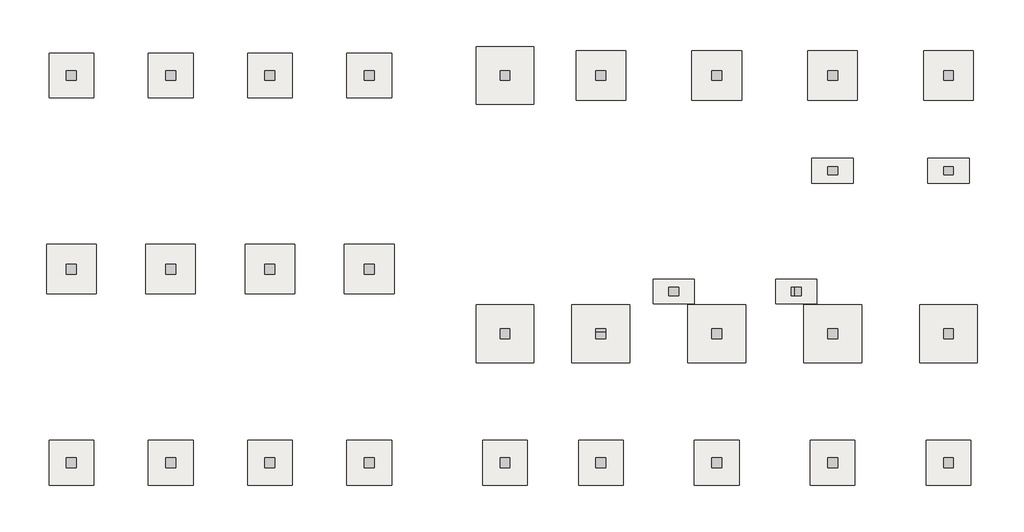
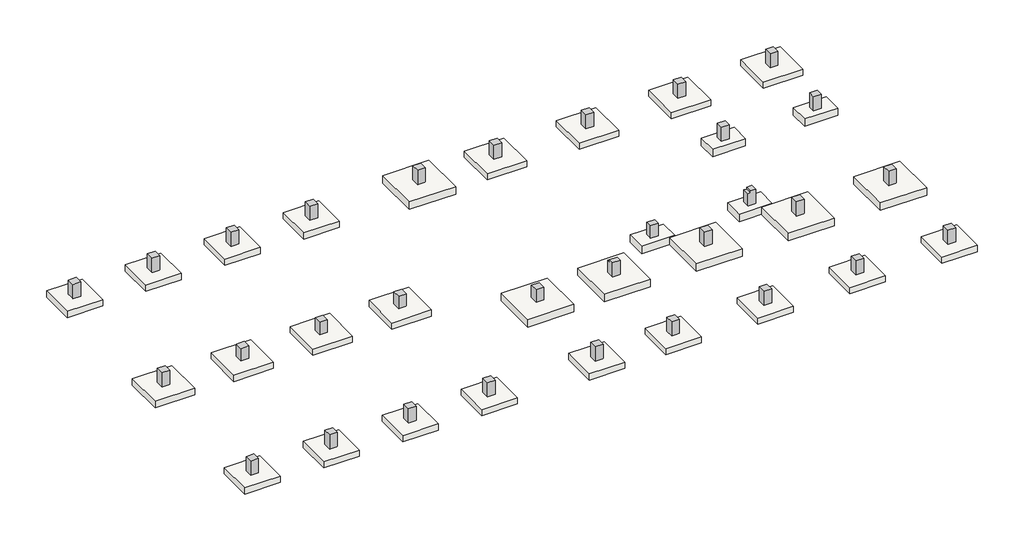
# Not in any storey: 31 columns, 31 slabs.
"""IFC4 building model written with IfcOpenShell, lengths in millimetres."""

import ifcopenshell
import ifcopenshell.guid

model = None  # the IFC model being written
_history = None  # IfcOwnerHistory: only IFC2X3 demands one
_inside = {}  # id of a spatial element -> (the spatial element, [elements in it])
_under = {}  # id of a project, library or spatial element -> (it, [spatial elements below it])
_declared = {}  # id of a project -> (the project, [libraries it declares])
_typed = {}  # id of a type object -> (the type object, [elements of that type])
_made_of = {}  # id of a material, layer set ... -> (it, [elements and type objects made of it])


def new_model(schema):
    """Start an empty IFC model of exactly this schema.

    Asked for "IFC4X3", IfcOpenShell would pick the latest addendum, in which some entities
    have other attributes; the version numbers below select the first issue.
    IFC2X3 requires an IfcOwnerHistory on every rooted entity: one is made here for all.
    """
    global model, _history
    if schema == "IFC4X3":
        model = ifcopenshell.file(schema_version=(4, 3, 0, 0))
    else:
        model = ifcopenshell.file(schema=schema)
    _inside.clear()
    _under.clear()
    _declared.clear()
    _typed.clear()
    _made_of.clear()
    _history = None
    if model.schema == "IFC2X3":
        org = make("IfcOrganization", Name="unknown")
        user = make(
            "IfcPersonAndOrganization",
            ThePerson=make("IfcPerson", FamilyName="unknown"),
            TheOrganization=org,
        )
        app = make(
            "IfcApplication",
            ApplicationDeveloper=org,
            Version="unknown",
            ApplicationFullName="unknown",
            ApplicationIdentifier="unknown",
        )
        _history = make(
            "IfcOwnerHistory",
            OwningUser=user,
            OwningApplication=app,
            ChangeAction="ADDED",
            CreationDate=0,
        )
    return model


def make(cls, **values):
    """One entity of the class cls with the attributes given. An attribute that is None is left unset."""
    return model.create_entity(
        cls, **{name: value for name, value in values.items() if value is not None}
    )


def rooted(cls, **values):
    """An entity with a GlobalId (a new one), such as an element, a storey or a relation."""
    return make(cls, GlobalId=ifcopenshell.guid.new(), OwnerHistory=_history, **values)


def si_unit(unit_type, name, prefix=None):
    """IfcSIUnit, for example si_unit("LENGTHUNIT", "METRE", prefix="MILLI")."""
    return make("IfcSIUnit", UnitType=unit_type, Prefix=prefix, Name=name)


def assignment(units):
    """IfcUnitAssignment: the units of a project."""
    return None if units is None else make("IfcUnitAssignment", Units=units)


def point(xyz):
    """IfcCartesianPoint."""
    return None if xyz is None else make("IfcCartesianPoint", Coordinates=xyz)


def direction(xyz):
    """IfcDirection."""
    return None if xyz is None else make("IfcDirection", DirectionRatios=xyz)


def frame(location, z_axis=None, x_axis=None):
    """IfcAxis2Placement3D, a coordinate frame: its origin and axes. An axis left out is left unset."""
    return make(
        "IfcAxis2Placement3D",
        Location=point(location),
        Axis=direction(z_axis),
        RefDirection=direction(x_axis),
    )


def origin():
    """The frame at (0, 0, 0) with its axes left unset."""
    return frame((0.0, 0.0, 0.0))


def place(relative_to, where):
    """IfcLocalPlacement: puts the frame where relative to a parent placement (None: the world)."""
    return make(
        "IfcLocalPlacement", PlacementRelTo=relative_to, RelativePlacement=where
    )


def context(
    kind, dimensions, precision=None, world=None, true_north=None, identifier=None
):
    """IfcGeometricRepresentationContext, for example the 3D "Model" context."""
    return make(
        "IfcGeometricRepresentationContext",
        ContextIdentifier=identifier,
        ContextType=kind,
        CoordinateSpaceDimension=dimensions,
        Precision=precision,
        WorldCoordinateSystem=world,
        TrueNorth=true_north,
    )


def project(units=None, contexts=None):
    """IfcProject with its units and contexts."""
    return rooted(
        "IfcProject",
        Name="project",
        RepresentationContexts=contexts,
        UnitsInContext=assignment(units),
    )


def spatial(cls, under=None, at=None, **own):
    """A site, building, storey or space (cls), placed at a placement, below another one or the project."""
    s = rooted(cls, ObjectPlacement=at, **own)
    if under is not None:
        _under.setdefault(under.id(), (under, []))[1].append(s)
    return s


def polyline(points):
    """IfcPolyline through the points."""
    return make("IfcPolyline", Points=[point(p) for p in points])


def outline(outer, holes=None, kind="AREA"):
    """IfcArbitraryClosedProfileDef: a profile drawn as a closed curve; with holes, ...WithVoids."""
    if holes is None:
        return make("IfcArbitraryClosedProfileDef", ProfileType=kind, OuterCurve=outer)
    return make(
        "IfcArbitraryProfileDefWithVoids",
        ProfileType=kind,
        OuterCurve=outer,
        InnerCurves=holes,
    )


def extrude(swept, where, along, depth):
    """IfcExtrudedAreaSolid: the profile swept, set in the frame where, extruded along a direction by depth."""
    return make(
        "IfcExtrudedAreaSolid",
        SweptArea=swept,
        Position=where,
        ExtrudedDirection=direction(along),
        Depth=depth,
    )


def faces_of(points, faces, orient=None, outer=None):
    """IfcFace entities. A face is a list of loops; a loop is a list of indices into points, from 0.

    orient and outer hold one flag for each loop. By default every Orientation is true, the
    first loop of a face is its IfcFaceOuterBound and the others are IfcFaceBound.
    """
    made = []
    for i, loops in enumerate(faces):
        bounds = []
        for j, loop in enumerate(loops):
            is_outer = j == 0 if outer is None else outer[i][j]
            bounds.append(
                make(
                    "IfcFaceOuterBound" if is_outer else "IfcFaceBound",
                    Bound=make("IfcPolyLoop", Polygon=[points[k] for k in loop]),
                    Orientation=True if orient is None else orient[i][j],
                )
            )
        made.append(make("IfcFace", Bounds=bounds))
    return made


def faceted_brep(points, faces, orient=None, outer=None, voids=None):
    """IfcFacetedBrep: a solid bounded by flat faces; with voids (closed shells), ...WithVoids."""
    shared = [point(p) for p in points]
    hull = make("IfcClosedShell", CfsFaces=faces_of(shared, faces, orient, outer))
    if voids is None:
        return make("IfcFacetedBrep", Outer=hull)
    return make(
        "IfcFacetedBrepWithVoids",
        Outer=hull,
        Voids=[
            make(cls, CfsFaces=faces_of(shared, fs, o, b)) for cls, fs, o, b in voids
        ],
    )


def shape(context_of_items, identifier, shape_type, items):
    """IfcShapeRepresentation: the items that make up one representation, for example the "Body"."""
    return make(
        "IfcShapeRepresentation",
        ContextOfItems=context_of_items,
        RepresentationIdentifier=identifier,
        RepresentationType=shape_type,
        Items=items,
    )


def made_of(thing, what):
    """Note that an element or type object is made of a material, layer set ...; save() writes the relation."""
    if what is not None:
        _made_of.setdefault(what.id(), (what, []))[1].append(thing)
    return thing


def element(
    cls,
    number,
    at=None,
    inside=None,
    cuts=None,
    type_object=None,
    material=None,
    context=None,
    identifier="Body",
    shape_type=None,
    held_by="IfcProductDefinitionShape",
    body=None,
    shapes=None,
    **own,
):
    """One element of the class cls, such as IfcWall. Its Tag is "e" and its number.

    at: its placement. inside: the storey or other place that contains it. cuts: it is an
    opening in that element (IfcRelVoidsElement). A single representation is given by context,
    identifier, shape_type and body (its items); several are given by shapes. held_by: the class
    of the entity that holds the representations. save() writes the other relations.
    """
    e = rooted(cls, Tag="e%d" % number, ObjectPlacement=at, **own)
    if body is not None:
        shapes = [shape(context, identifier, shape_type, body)]
    if shapes is not None:
        e.Representation = make(held_by, Representations=shapes)
    if inside is not None:
        _inside.setdefault(inside.id(), (inside, []))[1].append(e)
    if cuts is not None:
        rooted(
            "IfcRelVoidsElement", RelatingBuildingElement=cuts, RelatedOpeningElement=e
        )
    if type_object is not None:
        _typed.setdefault(type_object.id(), (type_object, []))[1].append(e)
    return made_of(e, material)


def aggregate(whole, parts):
    """IfcRelAggregates: a whole, such as a stair, and the parts it consists of."""
    return rooted("IfcRelAggregates", RelatingObject=whole, RelatedObjects=parts)


def save(model, path):
    """Write the relations noted so far, then the file.

    IfcRelAggregates (storeys below a building ...), IfcRelContainedInSpatialStructure (elements
    in a storey), IfcRelDefinesByType, IfcRelAssociatesMaterial and IfcRelDeclares: one each for
    every whole, place, type object, material and project.
    """
    for whole, parts in _under.values():
        aggregate(whole, parts)
    for where, things in _inside.values():
        rooted(
            "IfcRelContainedInSpatialStructure",
            RelatedElements=things,
            RelatingStructure=where,
        )
    for kind, things in _typed.values():
        rooted("IfcRelDefinesByType", RelatedObjects=things, RelatingType=kind)
    for what, things in _made_of.values():
        rooted("IfcRelAssociatesMaterial", RelatedObjects=things, RelatingMaterial=what)
    for by, libraries in _declared.values():
        rooted("IfcRelDeclares", RelatingContext=by, RelatedDefinitions=libraries)
    model.write(path)


model = new_model("IFC4")

# Units and contexts
model_context = context("Model", 3, world=origin())
ifc_project = project(units=[si_unit("LENGTHUNIT", "METRE", prefix="MILLI")], contexts=[model_context])

# Site, building
site = spatial("IfcSite", under=ifc_project)
building = spatial("IfcBuilding", under=site)

# Columns
placement = place(None, origin())
element("IfcColumn", 1, ObjectType="RC_Column_Rectangular : H_SC_AR_S15_UG PED_W600xL600_Bit", at=placement, inside=building, context=model_context, shape_type="Brep", body=[
    faceted_brep([(300.0, 12499.5208589, -1000.0381366), (300.0, 11899.5208589, -1000.0381366), (-300.0, 11899.5208589, -1000.0381366), (-300.0, 12499.5208589, -1000.0381366), (300.0, 12499.5208589, 149.9618634), (300.0, 11899.5208589, 149.9618634), (300.0, 11899.5208589, -0.0381366), (300.0, 11899.5208589, -500.0381366), (300.0, 12499.5208589, -500.0381366), (300.0, 12499.5208589, -0.0381366), (-300.0, 11899.5208589, 149.9618634), (-300.0, 11899.5208589, -0.0381366), (-300.0, 11899.5208589, -500.0381366), (-300.0, 12499.5208589, 149.9618634), (-300.0, 12499.5208589, -0.0381366), (-300.0, 12499.5208589, -500.0381366)], [[[0, 1, 2, 3]], [[4, 5, 6, 7, 1, 0, 8, 9]], [[5, 10, 11, 12, 2, 1, 7, 6]], [[10, 13, 14, 15, 3, 2, 12, 11]], [[13, 4, 9, 8, 0, 3, 15, 14]], [[4, 13, 10, 5]]]),
])
element("IfcColumn", 2, ObjectType="RC_Column_Rectangular : H_SC_AR_S15_UG PED_W600xL600_Bit", at=placement, inside=building, context=model_context, shape_type="SweptSolid", body=[
    extrude(outline(polyline([(6300.0, 12499.5208589), (6300.0, 11899.5208589), (5700.0, 11899.5208589), (5700.0, 12499.5208589), (6300.0, 12499.5208589)])), frame((0.0, 0.0, -1000.0381366), z_axis=(0.0, 0.0, 1.0), x_axis=(1.0, 0.0, 0.0)), (0.0, 0.0, 1.0), 1000.0),
])
element("IfcColumn", 3, ObjectType="RC_Column_Rectangular : H_SC_AR_S15_UG PED_W600xL600_Bit", at=placement, inside=building, context=model_context, shape_type="SweptSolid", body=[
    extrude(outline(polyline([(12300.0, 12499.5208589), (12300.0, 11899.5208589), (11700.0, 11899.5208589), (11700.0, 12499.5208589), (12300.0, 12499.5208589)])), frame((0.0, 0.0, -1000.0381366), z_axis=(0.0, 0.0, 1.0), x_axis=(1.0, 0.0, 0.0)), (0.0, 0.0, 1.0), 1000.0),
])
element("IfcColumn", 4, ObjectType="RC_Column_Rectangular : H_SC_AR_S15_UG PED_W600xL600_Bit", at=placement, inside=building, context=model_context, shape_type="Brep", body=[
    faceted_brep([(18300.0, 12499.5208589, -1000.0381366), (18300.0, 11899.5208589, -1000.0381366), (17700.0, 11899.5208589, -1000.0381366), (17700.0, 12499.5208589, -1000.0381366), (18300.0, 12499.5208589, -0.0381366), (18300.0, 11899.5208589, -0.0381366), (18200.0, 11899.5208589, -0.0381366), (17700.0, 11899.5208589, -0.0381366), (17700.0, 12499.5208589, -0.0381366)], [[[0, 1, 2, 3]], [[1, 0, 4, 5]], [[2, 1, 5, 6, 7]], [[3, 2, 7, 8]], [[0, 3, 8, 4]], [[5, 4, 8, 7, 6]]]),
])
element("IfcColumn", 5, ObjectType="RC_Column_Rectangular : H_SC_AR_S15_UG PED_W600xL600_Bit", at=placement, inside=building, context=model_context, shape_type="Brep", body=[
    faceted_brep([(300.0, 24199.5208589, -1000.0381366), (300.0, 23599.5208589, -1000.0381366), (-300.0, 23599.5208589, -1000.0381366), (-300.0, 24199.5208589, -1000.0381366), (300.0, 24199.5208589, 149.9618634), (300.0, 23599.5208589, 149.9618634), (300.0, 23599.5208589, -0.0381366), (300.0, 23599.5208589, -500.0381366), (300.0, 24199.5208589, -500.0381366), (300.0, 24199.5208589, -0.0381366), (-300.0, 23599.5208589, 149.9618634), (-300.0, 23599.5208589, -0.0381366), (-300.0, 23599.5208589, -500.0381366), (-300.0, 24199.5208589, 149.9618634)], [[[0, 1, 2, 3]], [[4, 5, 6, 7, 1, 0, 8, 9]], [[5, 10, 11, 12, 2, 1, 7, 6]], [[10, 13, 3, 2, 12, 11]], [[13, 4, 9, 8, 0, 3]], [[4, 13, 10, 5]]]),
])
element("IfcColumn", 6, ObjectType="RC_Column_Rectangular : H_SC_AR_S15_UG PED_W600xL600_Bit", at=placement, inside=building, context=model_context, shape_type="Brep", body=[
    faceted_brep([(6300.0, 24199.5208589, -1000.0381366), (6300.0, 23599.5208589, -1000.0381366), (5700.0, 23599.5208589, -1000.0381366), (5700.0, 24199.5208589, -1000.0381366), (6300.0, 24199.5208589, 149.9618634), (6300.0, 23599.5208589, 149.9618634), (6300.0, 23599.5208589, -0.0381366), (6300.0, 23599.5208589, -500.0381366), (6300.0, 24199.5208589, -500.0381366), (6300.0, 24199.5208589, -0.0381366), (5700.0, 23599.5208589, 149.9618634), (5700.0, 23599.5208589, -0.0381366), (5700.0, 23599.5208589, -500.0381366), (5700.0, 24199.5208589, 149.9618634), (5700.0, 24199.5208589, -0.0381366), (5700.0, 24199.5208589, -500.0381366)], [[[0, 1, 2, 3]], [[4, 5, 6, 7, 1, 0, 8, 9]], [[5, 10, 11, 12, 2, 1, 7, 6]], [[10, 13, 14, 15, 3, 2, 12, 11]], [[13, 4, 9, 8, 0, 3, 15, 14]], [[4, 13, 10, 5]]]),
])
element("IfcColumn", 7, ObjectType="RC_Column_Rectangular : H_SC_AR_S15_UG PED_W600xL600_Bit", at=placement, inside=building, context=model_context, shape_type="Brep", body=[
    faceted_brep([(12300.0, 24199.5208589, -1000.0381366), (12300.0, 23599.5208589, -1000.0381366), (11700.0, 23599.5208589, -1000.0381366), (11700.0, 24199.5208589, -1000.0381366), (12300.0, 24199.5208589, 149.9618634), (12300.0, 23599.5208589, 149.9618634), (12300.0, 23599.5208589, -0.0381366), (12300.0, 23599.5208589, -500.0381366), (12300.0, 24199.5208589, -500.0381366), (12300.0, 24199.5208589, -0.0381366), (11700.0, 23599.5208589, 149.9618634), (11700.0, 23599.5208589, -0.0381366), (11700.0, 23599.5208589, -500.0381366), (11700.0, 24199.5208589, 149.9618634), (11700.0, 24199.5208589, -0.0381366), (11700.0, 24199.5208589, -500.0381366)], [[[0, 1, 2, 3]], [[4, 5, 6, 7, 1, 0, 8, 9]], [[5, 10, 11, 12, 2, 1, 7, 6]], [[10, 13, 14, 15, 3, 2, 12, 11]], [[13, 4, 9, 8, 0, 3, 15, 14]], [[4, 13, 10, 5]]]),
])
element("IfcColumn", 8, ObjectType="RC_Column_Rectangular : H_SC_AR_S15_UG PED_W600xL600_Bit", at=placement, inside=building, context=model_context, shape_type="Brep", body=[
    faceted_brep([(18300.0, 24199.5208589, -1000.0381366), (18300.0, 23599.5208589, -1000.0381366), (17700.0, 23599.5208589, -1000.0381366), (17700.0, 24199.5208589, -1000.0381366), (18300.0, 24199.5208589, 149.9618634), (18300.0, 23599.5208589, 149.9618634), (18300.0, 23599.5208589, -0.0381366), (18300.0, 23599.5208589, -500.0381366), (18300.0, 24199.5208589, -500.0381366), (18300.0, 24199.5208589, -0.0381366), (17700.0, 23599.5208589, 149.9618634), (17700.0, 23599.5208589, -0.0381366), (17700.0, 23599.5208589, -500.0381366), (17700.0, 24199.5208589, 149.9618634), (17700.0, 24199.5208589, -0.0381366), (17700.0, 24199.5208589, -500.0381366)], [[[0, 1, 2, 3]], [[4, 5, 6, 7, 1, 0, 8, 9]], [[5, 10, 11, 12, 2, 1, 7, 6]], [[10, 13, 14, 15, 3, 2, 12, 11]], [[13, 4, 9, 8, 0, 3, 15, 14]], [[4, 13, 10, 5]]]),
])
element("IfcColumn", 9, ObjectType="RC_Column_Rectangular : H_SC_AR_S15_UG PED_W600xL600_Bit", at=placement, inside=building, context=model_context, shape_type="Brep", body=[
    faceted_brep([(26500.0, 24199.5208589, -1000.0381366), (26500.0, 23599.5208589, -1000.0381366), (25900.0, 23599.5208589, -1000.0381366), (25900.0, 24199.5208589, -1000.0381366), (26500.0, 24199.5208589, 149.9618634), (26500.0, 23599.5208589, 149.9618634), (26500.0, 23599.5208589, -0.0381366), (26500.0, 23599.5208589, -500.0381366), (26500.0, 24199.5208589, -500.0381366), (26500.0, 24199.5208589, -0.0381366), (25900.0, 23599.5208589, 149.9618634), (25900.0, 23599.5208589, -0.0381366), (25900.0, 23599.5208589, -500.0381366), (25900.0, 24199.5208589, 149.9618634), (25900.0, 24199.5208589, -0.0381366), (25900.0, 24199.5208589, -500.0381366)], [[[0, 1, 2, 3]], [[4, 5, 6, 7, 1, 0, 8, 9]], [[5, 10, 11, 12, 2, 1, 7, 6]], [[10, 13, 14, 15, 3, 2, 12, 11]], [[13, 4, 9, 8, 0, 3, 15, 14]], [[4, 13, 10, 5]]]),
])
element("IfcColumn", 10, ObjectType="RC_Column_Rectangular : H_SC_AR_S15_UG PED_W600xL600_Bit", at=placement, inside=building, context=model_context, shape_type="Brep", body=[
    faceted_brep([(32300.0, 24199.5208589, -1000.0381366), (32300.0, 23599.5208589, -1000.0381366), (31700.0, 23599.5208589, -1000.0381366), (31700.0, 24199.5208589, -1000.0381366), (32300.0, 24199.5208589, 149.9618634), (32300.0, 23599.5208589, 149.9618634), (32300.0, 23599.5208589, -0.0381366), (32300.0, 23599.5208589, -500.0381366), (32300.0, 24199.5208589, -500.0381366), (32300.0, 24199.5208589, -0.0381366), (31700.0, 23599.5208589, 149.9618634), (31700.0, 23599.5208589, -0.0381366), (31700.0, 23599.5208589, -500.0381366), (31700.0, 24199.5208589, 149.9618634), (31700.0, 24199.5208589, -0.0381366), (31700.0, 24199.5208589, -500.0381366)], [[[0, 1, 2, 3]], [[4, 5, 6, 7, 1, 0, 8, 9]], [[5, 10, 11, 12, 2, 1, 7, 6]], [[10, 13, 14, 15, 3, 2, 12, 11]], [[13, 4, 9, 8, 0, 3, 15, 14]], [[4, 13, 10, 5]]]),
])
element("IfcColumn", 11, ObjectType="RC_Column_Rectangular : H_SC_AR_S15_UG PED_W600xL600_Bit", at=placement, inside=building, context=model_context, shape_type="Brep", body=[
    faceted_brep([(39300.0, 24199.5208589, -1000.0381366), (39300.0, 23599.5208589, -1000.0381366), (38700.0, 23599.5208589, -1000.0381366), (38700.0, 24199.5208589, -1000.0381366), (39300.0, 24199.5208589, 149.9618634), (39300.0, 23599.5208589, 149.9618634), (39300.0, 23599.5208589, -0.0381366), (39300.0, 23599.5208589, -500.0381366), (39300.0, 24199.5208589, -500.0381366), (39300.0, 24199.5208589, -0.0381366), (38700.0, 23599.5208589, 149.9618634), (38700.0, 23599.5208589, -0.0381366), (38700.0, 23599.5208589, -500.0381366), (38700.0, 24199.5208589, 149.9618634), (38700.0, 24199.5208589, -0.0381366), (38700.0, 24199.5208589, -500.0381366)], [[[0, 1, 2, 3]], [[4, 5, 6, 7, 1, 0, 8, 9]], [[5, 10, 11, 12, 2, 1, 7, 6]], [[10, 13, 14, 15, 3, 2, 12, 11]], [[13, 4, 9, 8, 0, 3, 15, 14]], [[4, 13, 10, 5]]]),
])
element("IfcColumn", 12, ObjectType="RC_Column_Rectangular : H_SC_AR_S15_UG PED_W600xL600_Bit", at=placement, inside=building, context=model_context, shape_type="Brep", body=[
    faceted_brep([(46300.0, 24199.5208589, -1000.0381366), (46300.0, 23599.5208589, -1000.0381366), (45700.0, 23599.5208589, -1000.0381366), (45700.0, 24199.5208589, -1000.0381366), (46300.0, 24199.5208589, 149.9618634), (46300.0, 23599.5208589, 149.9618634), (46300.0, 23599.5208589, -0.0381366), (46300.0, 23599.5208589, -500.0381366), (46300.0, 24199.5208589, -500.0381366), (46300.0, 24199.5208589, -0.0381366), (45700.0, 23599.5208589, 149.9618634), (45700.0, 23599.5208589, -0.0381366), (45700.0, 23599.5208589, -500.0381366), (45700.0, 24199.5208589, 149.9618634), (45700.0, 24199.5208589, -0.0381366), (45700.0, 24199.5208589, -500.0381366)], [[[0, 1, 2, 3]], [[4, 5, 6, 7, 1, 0, 8, 9]], [[5, 10, 11, 12, 2, 1, 7, 6]], [[10, 13, 14, 15, 3, 2, 12, 11]], [[13, 4, 9, 8, 0, 3, 15, 14]], [[4, 13, 10, 5]]]),
])
element("IfcColumn", 13, ObjectType="RC_Column_Rectangular : H_SC_AR_S15_UG PED_W600xL600_Bit", at=placement, inside=building, context=model_context, shape_type="Brep", body=[
    faceted_brep([(53300.0, 24199.5208589, -1000.0381366), (53300.0, 23599.5208589, -1000.0381366), (52700.0, 23599.5208589, -1000.0381366), (52700.0, 24199.5208589, -1000.0381366), (53300.0, 24199.5208589, 149.9618634), (53300.0, 23599.5208589, 149.9618634), (53300.0, 23599.5208589, -0.0381366), (53300.0, 23599.5208589, -500.0381366), (52700.0, 23599.5208589, 149.9618634), (52700.0, 23599.5208589, -0.0381366), (52700.0, 23599.5208589, -500.0381366), (52700.0, 24199.5208589, 149.9618634), (52700.0, 24199.5208589, -0.0381366), (52700.0, 24199.5208589, -500.0381366)], [[[0, 1, 2, 3]], [[4, 5, 6, 7, 1, 0]], [[5, 8, 9, 10, 2, 1, 7, 6]], [[8, 11, 12, 13, 3, 2, 10, 9]], [[11, 4, 0, 3, 13, 12]], [[4, 11, 8, 5]]]),
])
element("IfcColumn", 14, ObjectType="RC_Column_Rectangular : H_SC_AR_S15_UG PED_W600xL600_Bit", at=placement, inside=building, context=model_context, shape_type="Brep", body=[
    faceted_brep([(26500.0, 8599.5208589, -1000.0381366), (26500.0, 7999.5208589, -1000.0381366), (25900.0, 7999.5208589, -1000.0381366), (25900.0, 8599.5208589, -1000.0381366), (26500.0, 8599.5208589, -0.0381366), (26500.0, 8399.5208589, -0.0381366), (26500.0, 7999.5208589, -0.0381366), (25900.0, 7999.5208589, -0.0381366), (25900.0, 8599.5208589, -0.0381366)], [[[0, 1, 2, 3]], [[1, 0, 4, 5, 6]], [[2, 1, 6, 7]], [[3, 2, 7, 8]], [[0, 3, 8, 4]], [[4, 8, 7, 6, 5]]]),
])
element("IfcColumn", 15, ObjectType="RC_Column_Rectangular : H_SC_AR_S15_UG PED_W600xL600_Bit", at=placement, inside=building, context=model_context, shape_type="Brep", body=[
    faceted_brep([(32300.0, 8599.5208589, -1000.0381366), (32300.0, 7999.5208589, -1000.0381366), (31700.0, 7999.5208589, -1000.0381366), (31700.0, 8599.5208589, -1000.0381366), (32300.0, 8599.5208589, -0.0381366), (32300.0, 8399.5208589, -0.0381366), (32300.0, 8399.5208589, 149.9618634), (32300.0, 7999.5208589, 149.9618634), (31700.0, 7999.5208589, 149.9618634), (31700.0, 8399.5208589, 149.9618634), (31700.0, 8399.5208589, -0.0381366), (31700.0, 8599.5208589, -0.0381366), (31800.0, 8399.5208589, 149.9618634), (31800.0, 8399.5208589, -0.0381366)], [[[0, 1, 2, 3]], [[1, 0, 4, 5, 6, 7]], [[2, 1, 7, 8]], [[3, 2, 8, 9, 10, 11]], [[0, 3, 11, 4]], [[8, 7, 6, 12, 9]], [[10, 13, 5, 4, 11]], [[5, 13, 12, 6]], [[13, 10, 9, 12]]]),
])
element("IfcColumn", 16, ObjectType="RC_Column_Rectangular : H_SC_AR_S15_UG PED_W600xL600_Bit", at=placement, inside=building, context=model_context, shape_type="SweptSolid", body=[
    extrude(outline(polyline([(39300.0, 8599.5208589), (39300.0, 7999.5208589), (38700.0, 7999.5208589), (38700.0, 8599.5208589), (39300.0, 8599.5208589)])), frame((0.0, 0.0, -1000.0381366), z_axis=(0.0, 0.0, 1.0), x_axis=(1.0, 0.0, 0.0)), (0.0, 0.0, 1.0), 1150.0),
])
element("IfcColumn", 17, ObjectType="RC_Column_Rectangular : H_SC_AR_S15_UG PED_W600xL600_Bit", at=placement, inside=building, context=model_context, shape_type="SweptSolid", body=[
    extrude(outline(polyline([(46300.0, 8599.5208589), (46300.0, 7999.5208589), (45700.0, 7999.5208589), (45700.0, 8599.5208589), (46300.0, 8599.5208589)])), frame((0.0, 0.0, -1000.0381366), z_axis=(0.0, 0.0, 1.0), x_axis=(1.0, 0.0, 0.0)), (0.0, 0.0, 1.0), 1150.0),
])
element("IfcColumn", 18, ObjectType="RC_Column_Rectangular : H_SC_AR_S15_UG PED_W600xL600_Bit", at=placement, inside=building, context=model_context, shape_type="Brep", body=[
    faceted_brep([(53300.0, 8599.5208589, -1000.0381366), (53300.0, 7999.5208589, -1000.0381366), (52700.0, 7999.5208589, -1000.0381366), (52700.0, 8599.5208589, -1000.0381366), (53300.0, 8599.5208589, 149.9618634), (53300.0, 7999.5208589, 149.9618634), (53300.0, 7999.5208589, -0.0381366), (53300.0, 7999.5208589, -500.0381366), (53300.0, 8599.5208589, -500.0381366), (53300.0, 8599.5208589, -0.0381366), (52700.0, 7999.5208589, 149.9618634), (52700.0, 7999.5208589, -0.0381366), (52700.0, 7999.5208589, -500.0381366), (52700.0, 8599.5208589, 149.9618634), (52700.0, 8599.5208589, -0.0381366), (52700.0, 8599.5208589, -500.0381366)], [[[0, 1, 2, 3]], [[4, 5, 6, 7, 1, 0, 8, 9]], [[5, 10, 11, 12, 2, 1, 7, 6]], [[10, 13, 14, 15, 3, 2, 12, 11]], [[13, 4, 9, 8, 0, 3, 15, 14]], [[4, 13, 10, 5]]]),
])
element("IfcColumn", 19, ObjectType="RC_Column_Rectangular : H_SC_AR_S15_UG PED_W600xL600_Bit", at=placement, inside=building, context=model_context, shape_type="Brep", body=[
    faceted_brep([(300.0, 799.5208589, -1000.0381366), (300.0, 199.5208589, -1000.0381366), (-300.0, 199.5208589, -1000.0381366), (-300.0, 799.5208589, -1000.0381366), (300.0, 799.5208589, 149.9618634), (300.0, 199.5208589, 149.9618634), (300.0, 199.5208589, -0.0381366), (300.0, 199.5208589, -500.0381366), (300.0, 799.5208589, -500.0381366), (300.0, 799.5208589, -0.0381366), (-300.0, 199.5208589, 149.9618634), (-300.0, 799.5208589, 149.9618634), (-300.0, 799.5208589, -0.0381366), (-300.0, 799.5208589, -500.0381366)], [[[0, 1, 2, 3]], [[4, 5, 6, 7, 1, 0, 8, 9]], [[5, 10, 2, 1, 7, 6]], [[10, 11, 12, 13, 3, 2]], [[11, 4, 9, 8, 0, 3, 13, 12]], [[4, 11, 10, 5]]]),
])
element("IfcColumn", 20, ObjectType="RC_Column_Rectangular : H_SC_AR_S15_UG PED_W600xL600_Bit", at=placement, inside=building, context=model_context, shape_type="Brep", body=[
    faceted_brep([(6300.0, 799.5208589, -1000.0381366), (6300.0, 199.5208589, -1000.0381366), (5700.0, 199.5208589, -1000.0381366), (5700.0, 799.5208589, -1000.0381366), (6300.0, 799.5208589, 149.9618634), (6300.0, 199.5208589, 149.9618634), (6300.0, 199.5208589, -0.0381366), (6300.0, 199.5208589, -500.0381366), (6300.0, 799.5208589, -500.0381366), (6300.0, 799.5208589, -0.0381366), (5700.0, 199.5208589, 149.9618634), (5700.0, 199.5208589, -0.0381366), (5700.0, 199.5208589, -500.0381366), (5700.0, 799.5208589, 149.9618634), (5700.0, 799.5208589, -0.0381366), (5700.0, 799.5208589, -500.0381366)], [[[0, 1, 2, 3]], [[4, 5, 6, 7, 1, 0, 8, 9]], [[5, 10, 11, 12, 2, 1, 7, 6]], [[10, 13, 14, 15, 3, 2, 12, 11]], [[13, 4, 9, 8, 0, 3, 15, 14]], [[4, 13, 10, 5]]]),
])
element("IfcColumn", 21, ObjectType="RC_Column_Rectangular : H_SC_AR_S15_UG PED_W600xL600_Bit", at=placement, inside=building, context=model_context, shape_type="Brep", body=[
    faceted_brep([(12300.0, 799.5208589, -1000.0381366), (12300.0, 199.5208589, -1000.0381366), (11700.0, 199.5208589, -1000.0381366), (11700.0, 799.5208589, -1000.0381366), (12300.0, 799.5208589, 149.9618634), (12300.0, 199.5208589, 149.9618634), (12300.0, 199.5208589, -0.0381366), (12300.0, 199.5208589, -500.0381366), (12300.0, 799.5208589, -500.0381366), (12300.0, 799.5208589, -0.0381366), (11700.0, 199.5208589, 149.9618634), (11700.0, 199.5208589, -0.0381366), (11700.0, 199.5208589, -500.0381366), (11700.0, 799.5208589, 149.9618634), (11700.0, 799.5208589, -0.0381366), (11700.0, 799.5208589, -500.0381366)], [[[0, 1, 2, 3]], [[4, 5, 6, 7, 1, 0, 8, 9]], [[5, 10, 11, 12, 2, 1, 7, 6]], [[10, 13, 14, 15, 3, 2, 12, 11]], [[13, 4, 9, 8, 0, 3, 15, 14]], [[4, 13, 10, 5]]]),
])
element("IfcColumn", 22, ObjectType="RC_Column_Rectangular : H_SC_AR_S15_UG PED_W600xL600_Bit", at=placement, inside=building, context=model_context, shape_type="Brep", body=[
    faceted_brep([(18300.0, 799.5208589, -1000.0381366), (18300.0, 199.5208589, -1000.0381366), (17700.0, 199.5208589, -1000.0381366), (17700.0, 799.5208589, -1000.0381366), (18300.0, 799.5208589, 149.9618634), (18300.0, 199.5208589, 149.9618634), (18300.0, 199.5208589, -0.0381366), (18300.0, 199.5208589, -500.0381366), (18300.0, 799.5208589, -500.0381366), (18300.0, 799.5208589, -0.0381366), (17700.0, 199.5208589, 149.9618634), (17700.0, 199.5208589, -0.0381366), (17700.0, 199.5208589, -500.0381366), (17700.0, 799.5208589, 149.9618634), (17700.0, 799.5208589, -0.0381366), (17700.0, 799.5208589, -500.0381366)], [[[0, 1, 2, 3]], [[4, 5, 6, 7, 1, 0, 8, 9]], [[5, 10, 11, 12, 2, 1, 7, 6]], [[10, 13, 14, 15, 3, 2, 12, 11]], [[13, 4, 9, 8, 0, 3, 15, 14]], [[4, 13, 10, 5]]]),
])
element("IfcColumn", 23, ObjectType="RC_Column_Rectangular : H_SC_AR_S15_UG PED_W600xL600_Bit", at=placement, inside=building, context=model_context, shape_type="Brep", body=[
    faceted_brep([(26500.0, 799.5208589, -1000.0381366), (26500.0, 199.5208589, -1000.0381366), (25900.0, 199.5208589, -1000.0381366), (25900.0, 799.5208589, -1000.0381366), (26500.0, 799.5208589, 149.9618634), (26500.0, 199.5208589, 149.9618634), (26500.0, 199.5208589, -0.0381366), (26500.0, 199.5208589, -500.0381366), (26500.0, 799.5208589, -500.0381366), (26500.0, 799.5208589, -0.0381366), (25900.0, 199.5208589, 149.9618634), (25900.0, 199.5208589, -0.0381366), (25900.0, 199.5208589, -500.0381366), (25900.0, 799.5208589, 149.9618634), (25900.0, 799.5208589, -0.0381366), (25900.0, 799.5208589, -500.0381366)], [[[0, 1, 2, 3]], [[4, 5, 6, 7, 1, 0, 8, 9]], [[5, 10, 11, 12, 2, 1, 7, 6]], [[10, 13, 14, 15, 3, 2, 12, 11]], [[13, 4, 9, 8, 0, 3, 15, 14]], [[4, 13, 10, 5]]]),
])
element("IfcColumn", 24, ObjectType="RC_Column_Rectangular : H_SC_AR_S15_UG PED_W600xL600_Bit", at=placement, inside=building, context=model_context, shape_type="Brep", body=[
    faceted_brep([(32300.0, 799.5208589, -1000.0381366), (32300.0, 199.5208589, -1000.0381366), (31700.0, 199.5208589, -1000.0381366), (31700.0, 799.5208589, -1000.0381366), (32300.0, 799.5208589, 149.9618634), (32300.0, 199.5208589, 149.9618634), (32300.0, 199.5208589, -0.0381366), (32300.0, 199.5208589, -500.0381366), (32300.0, 799.5208589, -500.0381366), (32300.0, 799.5208589, -0.0381366), (31700.0, 199.5208589, 149.9618634), (31700.0, 199.5208589, -0.0381366), (31700.0, 199.5208589, -500.0381366), (31700.0, 799.5208589, 149.9618634), (31700.0, 799.5208589, -0.0381366), (31700.0, 799.5208589, -500.0381366)], [[[0, 1, 2, 3]], [[4, 5, 6, 7, 1, 0, 8, 9]], [[5, 10, 11, 12, 2, 1, 7, 6]], [[10, 13, 14, 15, 3, 2, 12, 11]], [[13, 4, 9, 8, 0, 3, 15, 14]], [[4, 13, 10, 5]]]),
])
element("IfcColumn", 25, ObjectType="RC_Column_Rectangular : H_SC_AR_S15_UG PED_W600xL600_Bit", at=placement, inside=building, context=model_context, shape_type="Brep", body=[
    faceted_brep([(39300.0, 799.5208589, -1000.0381366), (39300.0, 199.5208589, -1000.0381366), (38700.0, 199.5208589, -1000.0381366), (38700.0, 799.5208589, -1000.0381366), (39300.0, 799.5208589, 149.9618634), (39300.0, 199.5208589, 149.9618634), (39300.0, 199.5208589, -0.0381366), (39300.0, 199.5208589, -500.0381366), (39300.0, 799.5208589, -500.0381366), (39300.0, 799.5208589, -0.0381366), (38700.0, 199.5208589, 149.9618634), (38700.0, 199.5208589, -0.0381366), (38700.0, 199.5208589, -500.0381366), (38700.0, 799.5208589, 149.9618634), (38700.0, 799.5208589, -0.0381366), (38700.0, 799.5208589, -500.0381366)], [[[0, 1, 2, 3]], [[4, 5, 6, 7, 1, 0, 8, 9]], [[5, 10, 11, 12, 2, 1, 7, 6]], [[10, 13, 14, 15, 3, 2, 12, 11]], [[13, 4, 9, 8, 0, 3, 15, 14]], [[4, 13, 10, 5]]]),
])
element("IfcColumn", 26, ObjectType="RC_Column_Rectangular : H_SC_AR_S15_UG PED_W600xL600_Bit", at=placement, inside=building, context=model_context, shape_type="Brep", body=[
    faceted_brep([(46300.0, 799.5208589, -1000.0381366), (46300.0, 199.5208589, -1000.0381366), (45700.0, 199.5208589, -1000.0381366), (45700.0, 799.5208589, -1000.0381366), (46300.0, 799.5208589, 149.9618634), (46300.0, 199.5208589, 149.9618634), (46300.0, 199.5208589, -0.0381366), (46300.0, 199.5208589, -500.0381366), (46300.0, 799.5208589, -500.0381366), (46300.0, 799.5208589, -0.0381366), (45700.0, 199.5208589, 149.9618634), (45700.0, 199.5208589, -0.0381366), (45700.0, 199.5208589, -500.0381366), (45700.0, 799.5208589, 149.9618634), (45700.0, 799.5208589, -0.0381366), (45700.0, 799.5208589, -500.0381366)], [[[0, 1, 2, 3]], [[4, 5, 6, 7, 1, 0, 8, 9]], [[5, 10, 11, 12, 2, 1, 7, 6]], [[10, 13, 14, 15, 3, 2, 12, 11]], [[13, 4, 9, 8, 0, 3, 15, 14]], [[4, 13, 10, 5]]]),
])
element("IfcColumn", 27, ObjectType="RC_Column_Rectangular : H_SC_AR_S15_UG PED_W600xL600_Bit", at=placement, inside=building, context=model_context, shape_type="Brep", body=[
    faceted_brep([(53300.0, 799.5208589, -1000.0381366), (53300.0, 199.5208589, -1000.0381366), (52700.0, 199.5208589, -1000.0381366), (52700.0, 799.5208589, -1000.0381366), (53300.0, 799.5208589, 149.9618634), (53300.0, 199.5208589, 149.9618634), (53300.0, 799.5208589, -500.0381366), (53300.0, 799.5208589, -0.0381366), (52700.0, 199.5208589, 149.9618634), (52700.0, 199.5208589, -0.0381366), (52700.0, 199.5208589, -500.0381366), (52700.0, 799.5208589, 149.9618634), (52700.0, 799.5208589, -0.0381366), (52700.0, 799.5208589, -500.0381366)], [[[0, 1, 2, 3]], [[4, 5, 1, 0, 6, 7]], [[5, 8, 9, 10, 2, 1]], [[8, 11, 12, 13, 3, 2, 10, 9]], [[11, 4, 7, 6, 0, 3, 13, 12]], [[4, 11, 8, 5]]]),
])
element("IfcColumn", 28, ObjectType="RC_Column_Rectangular : H_SC_AR_S15_UG PED_W600xL500_Bit_PD1A", at=placement, inside=building, context=model_context, shape_type="Brep", body=[
    faceted_brep([(52700.0, 18399.5208589, -1000.0381366), (53300.0, 18399.5208589, -1000.0381366), (53300.0, 17899.5208589, -1000.0381366), (52700.0, 17899.5208589, -1000.0381366), (52700.0, 18399.5208589, 149.9618634), (53300.0, 18399.5208589, 149.9618634), (53300.0, 18399.5208589, -0.0381366), (53300.0, 18399.5208589, -500.0381366), (52700.0, 18399.5208589, -500.0381366), (52700.0, 18399.5208589, -0.0381366), (53300.0, 17899.5208589, 149.9618634), (53300.0, 17899.5208589, -0.0381366), (53300.0, 17899.5208589, -500.0381366), (52700.0, 17899.5208589, 149.9618634), (52700.0, 17899.5208589, -0.0381366), (52700.0, 17899.5208589, -500.0381366)], [[[0, 1, 2, 3]], [[4, 5, 6, 7, 1, 0, 8, 9]], [[5, 10, 11, 12, 2, 1, 7, 6]], [[10, 13, 14, 15, 3, 2, 12, 11]], [[13, 4, 9, 8, 0, 3, 15, 14]], [[4, 13, 10, 5]]]),
])
element("IfcColumn", 29, ObjectType="RC_Column_Rectangular : H_SC_AR_S15_UG PED_W600xL500_Bit_PD1A", at=placement, inside=building, context=model_context, shape_type="SweptSolid", body=[
    extrude(outline(polyline([(45700.0, 18399.5208589), (46300.0, 18399.5208589), (46300.0, 17899.5208589), (45700.0, 17899.5208589), (45700.0, 18399.5208589)])), frame((0.0, 0.0, -1000.0381366), z_axis=(0.0, 0.0, 1.0), x_axis=(1.0, 0.0, 0.0)), (0.0, 0.0, 1.0), 1150.0),
])
element("IfcColumn", 30, ObjectType="RC_Column_Rectangular : H_SC_AR_S15_UG PED_W600xL500_Bit_PD1A", at=placement, inside=building, context=model_context, shape_type="SweptSolid", body=[
    extrude(outline(polyline([(36100.0, 11099.5208589), (36700.0, 11099.5208589), (36700.0, 10599.5208589), (36100.0, 10599.5208589), (36100.0, 11099.5208589)])), frame((0.0, 0.0, -1000.0381366), z_axis=(0.0, 0.0, 1.0), x_axis=(1.0, 0.0, 0.0)), (0.0, 0.0, 1.0), 1000.0),
])
element("IfcColumn", 31, ObjectType="RC_Column_Rectangular : H_SC_AR_S15_UG PED_W600xL500_Bit_PD1A", at=placement, inside=building, context=model_context, shape_type="SweptSolid", body=[
    extrude(outline(polyline([(-1000.0381366, 43500.0), (-1000.0381366, 44100.0), (149.9618634, 44100.0), (149.9618634, 43700.0), (-0.0381366, 43700.0), (-0.0381366, 43500.0), (-1000.0381366, 43500.0)])), frame((0.0, 10599.5208589, 0.0), z_axis=(0.0, 1.0, 0.0), x_axis=(0.0, 0.0, 1.0)), (0.0, 0.0, 1.0), 500.0),
])

# Slabs
element("IfcSlab", 32, ObjectType="Foundation Rectangular (Non-Pile) : H_SF_AR_S18_W3000xL3000xT500_Bitumen_F2", at=placement, inside=building, context=model_context, shape_type="SweptSolid", body=[
    extrude(outline(polyline([(1500.0, 13699.5208589), (1500.0, 10699.5208589), (-1500.0, 10699.5208589), (-1500.0, 13699.5208589), (1500.0, 13699.5208589)])), frame((0.0, 0.0, -1500.0381366), z_axis=(0.0, 0.0, 1.0), x_axis=(1.0, 0.0, 0.0)), (0.0, 0.0, 1.0), 500.0),
])
element("IfcSlab", 33, ObjectType="Foundation Rectangular (Non-Pile) : H_SF_AR_S18_W3000xL3000xT500_Bitumen_F2", at=placement, inside=building, context=model_context, shape_type="SweptSolid", body=[
    extrude(outline(polyline([(7500.0, 13699.5208589), (7500.0, 10699.5208589), (4500.0, 10699.5208589), (4500.0, 13699.5208589), (7500.0, 13699.5208589)])), frame((0.0, 0.0, -1500.0381366), z_axis=(0.0, 0.0, 1.0), x_axis=(1.0, 0.0, 0.0)), (0.0, 0.0, 1.0), 500.0),
])
element("IfcSlab", 34, ObjectType="Foundation Rectangular (Non-Pile) : H_SF_AR_S18_W3000xL3000xT500_Bitumen_F2", at=placement, inside=building, context=model_context, shape_type="SweptSolid", body=[
    extrude(outline(polyline([(13500.0, 13699.5208589), (13500.0, 10699.5208589), (10500.0, 10699.5208589), (10500.0, 13699.5208589), (13500.0, 13699.5208589)])), frame((0.0, 0.0, -1500.0381366), z_axis=(0.0, 0.0, 1.0), x_axis=(1.0, 0.0, 0.0)), (0.0, 0.0, 1.0), 500.0),
])
element("IfcSlab", 35, ObjectType="Foundation Rectangular (Non-Pile) : H_SF_AR_S18_W3000xL3000xT500_Bitumen_F2", at=placement, inside=building, context=model_context, shape_type="SweptSolid", body=[
    extrude(outline(polyline([(19500.0, 13699.5208589), (19500.0, 10699.5208589), (16500.0, 10699.5208589), (16500.0, 13699.5208589), (19500.0, 13699.5208589)])), frame((0.0, 0.0, -1500.0381366), z_axis=(0.0, 0.0, 1.0), x_axis=(1.0, 0.0, 0.0)), (0.0, 0.0, 1.0), 500.0),
])
element("IfcSlab", 36, ObjectType="Foundation Rectangular (Non-Pile) : H_SF_AR_S18_W2700xL2700xT500_Bitumen_F1", at=placement, inside=building, context=model_context, shape_type="SweptSolid", body=[
    extrude(outline(polyline([(1350.0, 25249.5208589), (1350.0, 22549.5208589), (-1350.0, 22549.5208589), (-1350.0, 25249.5208589), (1350.0, 25249.5208589)])), frame((0.0, 0.0, -1500.0381366), z_axis=(0.0, 0.0, 1.0), x_axis=(1.0, 0.0, 0.0)), (0.0, 0.0, 1.0), 500.0),
])
element("IfcSlab", 37, ObjectType="Foundation Rectangular (Non-Pile) : H_SF_AR_S18_W2700xL2700xT500_Bitumen_F1", at=placement, inside=building, context=model_context, shape_type="SweptSolid", body=[
    extrude(outline(polyline([(7350.0, 25249.5208589), (7350.0, 22549.5208589), (4650.0, 22549.5208589), (4650.0, 25249.5208589), (7350.0, 25249.5208589)])), frame((0.0, 0.0, -1500.0381366), z_axis=(0.0, 0.0, 1.0), x_axis=(1.0, 0.0, 0.0)), (0.0, 0.0, 1.0), 500.0),
])
element("IfcSlab", 38, ObjectType="Foundation Rectangular (Non-Pile) : H_SF_AR_S18_W2700xL2700xT500_Bitumen_F1", at=placement, inside=building, context=model_context, shape_type="SweptSolid", body=[
    extrude(outline(polyline([(13350.0, 25249.5208589), (13350.0, 22549.5208589), (10650.0, 22549.5208589), (10650.0, 25249.5208589), (13350.0, 25249.5208589)])), frame((0.0, 0.0, -1500.0381366), z_axis=(0.0, 0.0, 1.0), x_axis=(1.0, 0.0, 0.0)), (0.0, 0.0, 1.0), 500.0),
])
element("IfcSlab", 39, ObjectType="Foundation Rectangular (Non-Pile) : H_SF_AR_S18_W2700xL2700xT500_Bitumen_F1", at=placement, inside=building, context=model_context, shape_type="SweptSolid", body=[
    extrude(outline(polyline([(19350.0, 25249.5208589), (19350.0, 22549.5208589), (16650.0, 22549.5208589), (16650.0, 25249.5208589), (19350.0, 25249.5208589)])), frame((0.0, 0.0, -1500.0381366), z_axis=(0.0, 0.0, 1.0), x_axis=(1.0, 0.0, 0.0)), (0.0, 0.0, 1.0), 500.0),
])
element("IfcSlab", 40, ObjectType="Foundation Rectangular (Non-Pile) : H_SF_AR_S18_W3500xL3500xT600_Bitumen_F3", at=placement, inside=building, context=model_context, shape_type="SweptSolid", body=[
    extrude(outline(polyline([(27950.0, 25649.5208589), (27950.0, 22149.5208589), (24450.0, 22149.5208589), (24450.0, 25649.5208589), (27950.0, 25649.5208589)])), frame((0.0, 0.0, -1600.0381366), z_axis=(0.0, 0.0, 1.0), x_axis=(1.0, 0.0, 0.0)), (0.0, 0.0, 1.0), 600.0),
])
element("IfcSlab", 41, ObjectType="Foundation Rectangular (Non-Pile) : H_SF_AR_S18_W3000xL3000xT500_Bitumen_F2A", at=placement, inside=building, context=model_context, shape_type="SweptSolid", body=[
    extrude(outline(polyline([(33500.0, 25399.5208589), (33500.0, 22399.5208589), (30500.0, 22399.5208589), (30500.0, 25399.5208589), (33500.0, 25399.5208589)])), frame((0.0, 0.0, -1500.0381366), z_axis=(0.0, 0.0, 1.0), x_axis=(1.0, 0.0, 0.0)), (0.0, 0.0, 1.0), 500.0),
])
element("IfcSlab", 42, ObjectType="Foundation Rectangular (Non-Pile) : H_SF_AR_S18_W3000xL3000xT500_Bitumen_F2A", at=placement, inside=building, context=model_context, shape_type="SweptSolid", body=[
    extrude(outline(polyline([(40500.0, 25399.5208589), (40500.0, 22399.5208589), (37500.0, 22399.5208589), (37500.0, 25399.5208589), (40500.0, 25399.5208589)])), frame((0.0, 0.0, -1500.0381366), z_axis=(0.0, 0.0, 1.0), x_axis=(1.0, 0.0, 0.0)), (0.0, 0.0, 1.0), 500.0),
])
element("IfcSlab", 43, ObjectType="Foundation Rectangular (Non-Pile) : H_SF_AR_S18_W3000xL3000xT500_Bitumen_F2A", at=placement, inside=building, context=model_context, shape_type="SweptSolid", body=[
    extrude(outline(polyline([(47500.0, 25399.5208589), (47500.0, 22399.5208589), (44500.0, 22399.5208589), (44500.0, 25399.5208589), (47500.0, 25399.5208589)])), frame((0.0, 0.0, -1500.0381366), z_axis=(0.0, 0.0, 1.0), x_axis=(1.0, 0.0, 0.0)), (0.0, 0.0, 1.0), 500.0),
])
element("IfcSlab", 44, ObjectType="Foundation Rectangular (Non-Pile) : H_SF_AR_S18_W3000xL3000xT500_Bitumen_F2A", at=placement, inside=building, context=model_context, shape_type="SweptSolid", body=[
    extrude(outline(polyline([(54500.0, 25399.5208589), (54500.0, 22399.5208589), (51500.0, 22399.5208589), (51500.0, 25399.5208589), (54500.0, 25399.5208589)])), frame((0.0, 0.0, -1500.0381366), z_axis=(0.0, 0.0, 1.0), x_axis=(1.0, 0.0, 0.0)), (0.0, 0.0, 1.0), 500.0),
])
element("IfcSlab", 45, ObjectType="Foundation Rectangular (Non-Pile) : H_SF_AR_S18_W3500xL3500xT600_Bitumen_F3", at=placement, inside=building, context=model_context, shape_type="SweptSolid", body=[
    extrude(outline(polyline([(27950.0, 10049.5208589), (27950.0, 6549.5208589), (24450.0, 6549.5208589), (24450.0, 10049.5208589), (27950.0, 10049.5208589)])), frame((0.0, 0.0, -1600.0381366), z_axis=(0.0, 0.0, 1.0), x_axis=(1.0, 0.0, 0.0)), (0.0, 0.0, 1.0), 600.0),
])
element("IfcSlab", 46, ObjectType="Foundation Rectangular (Non-Pile) : H_SF_AR_S18_W3500xL3500xT600_Bitumen_F3", at=placement, inside=building, context=model_context, shape_type="SweptSolid", body=[
    extrude(outline(polyline([(33750.0, 10049.5208589), (33750.0, 6549.5208589), (30250.0, 6549.5208589), (30250.0, 10049.5208589), (33750.0, 10049.5208589)])), frame((0.0, 0.0, -1600.0381366), z_axis=(0.0, 0.0, 1.0), x_axis=(1.0, 0.0, 0.0)), (0.0, 0.0, 1.0), 600.0),
])
element("IfcSlab", 47, ObjectType="Foundation Rectangular (Non-Pile) : H_SF_AR_S18_W3500xL3500xT600_Bitumen_F3", at=placement, inside=building, context=model_context, shape_type="SweptSolid", body=[
    extrude(outline(polyline([(40750.0, 10049.5208589), (40750.0, 6549.5208589), (37250.0, 6549.5208589), (37250.0, 10049.5208589), (40750.0, 10049.5208589)])), frame((0.0, 0.0, -1600.0381366), z_axis=(0.0, 0.0, 1.0), x_axis=(1.0, 0.0, 0.0)), (0.0, 0.0, 1.0), 600.0),
])
element("IfcSlab", 48, ObjectType="Foundation Rectangular (Non-Pile) : H_SF_AR_S18_W3500xL3500xT600_Bitumen_F3", at=placement, inside=building, context=model_context, shape_type="SweptSolid", body=[
    extrude(outline(polyline([(47750.0, 10049.5208589), (47750.0, 6549.5208589), (44250.0, 6549.5208589), (44250.0, 10049.5208589), (47750.0, 10049.5208589)])), frame((0.0, 0.0, -1600.0381366), z_axis=(0.0, 0.0, 1.0), x_axis=(1.0, 0.0, 0.0)), (0.0, 0.0, 1.0), 600.0),
])
element("IfcSlab", 49, ObjectType="Foundation Rectangular (Non-Pile) : H_SF_AR_S18_W3500xL3500xT600_Bitumen_F3", at=placement, inside=building, context=model_context, shape_type="SweptSolid", body=[
    extrude(outline(polyline([(54750.0, 10049.5208589), (54750.0, 6549.5208589), (51250.0, 6549.5208589), (51250.0, 10049.5208589), (54750.0, 10049.5208589)])), frame((0.0, 0.0, -1600.0381366), z_axis=(0.0, 0.0, 1.0), x_axis=(1.0, 0.0, 0.0)), (0.0, 0.0, 1.0), 600.0),
])
element("IfcSlab", 50, ObjectType="Foundation Rectangular (Non-Pile) : H_SF_AR_S18_W2700xL2700xT500_Bitumen_F1A", at=placement, inside=building, context=model_context, shape_type="SweptSolid", body=[
    extrude(outline(polyline([(1350.0, 1849.5208589), (1350.0, -850.4791411), (-1350.0, -850.4791411), (-1350.0, 1849.5208589), (1350.0, 1849.5208589)])), frame((0.0, 0.0, -1500.0381366), z_axis=(0.0, 0.0, 1.0), x_axis=(1.0, 0.0, 0.0)), (0.0, 0.0, 1.0), 500.0),
])
element("IfcSlab", 51, ObjectType="Foundation Rectangular (Non-Pile) : H_SF_AR_S18_W2700xL2700xT500_Bitumen_F1", at=placement, inside=building, context=model_context, shape_type="SweptSolid", body=[
    extrude(outline(polyline([(7350.0, 1849.5208589), (7350.0, -850.4791411), (4650.0, -850.4791411), (4650.0, 1849.5208589), (7350.0, 1849.5208589)])), frame((0.0, 0.0, -1500.0381366), z_axis=(0.0, 0.0, 1.0), x_axis=(1.0, 0.0, 0.0)), (0.0, 0.0, 1.0), 500.0),
])
element("IfcSlab", 52, ObjectType="Foundation Rectangular (Non-Pile) : H_SF_AR_S18_W2700xL2700xT500_Bitumen_F1", at=placement, inside=building, context=model_context, shape_type="SweptSolid", body=[
    extrude(outline(polyline([(13350.0, 1849.5208589), (13350.0, -850.4791411), (10650.0, -850.4791411), (10650.0, 1849.5208589), (13350.0, 1849.5208589)])), frame((0.0, 0.0, -1500.0381366), z_axis=(0.0, 0.0, 1.0), x_axis=(1.0, 0.0, 0.0)), (0.0, 0.0, 1.0), 500.0),
])
element("IfcSlab", 53, ObjectType="Foundation Rectangular (Non-Pile) : H_SF_AR_S18_W2700xL2700xT500_Bitumen_F1", at=placement, inside=building, context=model_context, shape_type="SweptSolid", body=[
    extrude(outline(polyline([(19350.0, 1849.5208589), (19350.0, -850.4791411), (16650.0, -850.4791411), (16650.0, 1849.5208589), (19350.0, 1849.5208589)])), frame((0.0, 0.0, -1500.0381366), z_axis=(0.0, 0.0, 1.0), x_axis=(1.0, 0.0, 0.0)), (0.0, 0.0, 1.0), 500.0),
])
element("IfcSlab", 54, ObjectType="Foundation Rectangular (Non-Pile) : H_SF_AR_S18_W2700xL2700xT500_Bitumen_F1A", at=placement, inside=building, context=model_context, shape_type="SweptSolid", body=[
    extrude(outline(polyline([(27550.0, 1849.5208589), (27550.0, -850.4791411), (24850.0, -850.4791411), (24850.0, 1849.5208589), (27550.0, 1849.5208589)])), frame((0.0, 0.0, -1500.0381366), z_axis=(0.0, 0.0, 1.0), x_axis=(1.0, 0.0, 0.0)), (0.0, 0.0, 1.0), 500.0),
])
element("IfcSlab", 55, ObjectType="Foundation Rectangular (Non-Pile) : H_SF_AR_S18_W2700xL2700xT500_Bitumen_F1A", at=placement, inside=building, context=model_context, shape_type="SweptSolid", body=[
    extrude(outline(polyline([(33350.0, 1849.5208589), (33350.0, -850.4791411), (30650.0, -850.4791411), (30650.0, 1849.5208589), (33350.0, 1849.5208589)])), frame((0.0, 0.0, -1500.0381366), z_axis=(0.0, 0.0, 1.0), x_axis=(1.0, 0.0, 0.0)), (0.0, 0.0, 1.0), 500.0),
])
element("IfcSlab", 56, ObjectType="Foundation Rectangular (Non-Pile) : H_SF_AR_S18_W2700xL2700xT500_Bitumen_F1", at=placement, inside=building, context=model_context, shape_type="SweptSolid", body=[
    extrude(outline(polyline([(40350.0, 1849.5208589), (40350.0, -850.4791411), (37650.0, -850.4791411), (37650.0, 1849.5208589), (40350.0, 1849.5208589)])), frame((0.0, 0.0, -1500.0381366), z_axis=(0.0, 0.0, 1.0), x_axis=(1.0, 0.0, 0.0)), (0.0, 0.0, 1.0), 500.0),
])
element("IfcSlab", 57, ObjectType="Foundation Rectangular (Non-Pile) : H_SF_AR_S18_W2700xL2700xT500_Bitumen_F1", at=placement, inside=building, context=model_context, shape_type="SweptSolid", body=[
    extrude(outline(polyline([(47350.0, 1849.5208589), (47350.0, -850.4791411), (44650.0, -850.4791411), (44650.0, 1849.5208589), (47350.0, 1849.5208589)])), frame((0.0, 0.0, -1500.0381366), z_axis=(0.0, 0.0, 1.0), x_axis=(1.0, 0.0, 0.0)), (0.0, 0.0, 1.0), 500.0),
])
element("IfcSlab", 58, ObjectType="Foundation Rectangular (Non-Pile) : H_SF_AR_S18_W2700xL2700xT500_Bitumen_F1", at=placement, inside=building, context=model_context, shape_type="SweptSolid", body=[
    extrude(outline(polyline([(54350.0, 1849.5208589), (54350.0, -850.4791411), (51650.0, -850.4791411), (51650.0, 1849.5208589), (54350.0, 1849.5208589)])), frame((0.0, 0.0, -1500.0381366), z_axis=(0.0, 0.0, 1.0), x_axis=(1.0, 0.0, 0.0)), (0.0, 0.0, 1.0), 500.0),
])
element("IfcSlab", 59, ObjectType="Foundation Rectangular (Non-Pile) : H_SF_AR_S18_W2500xL1500xT600_Bitumen_F4", at=placement, inside=building, context=model_context, shape_type="SweptSolid", body=[
    extrude(outline(polyline([(47250.0, 18899.5208589), (47250.0, 17399.5208589), (44750.0, 17399.5208589), (44750.0, 18899.5208589), (47250.0, 18899.5208589)])), frame((0.0, 0.0, -1600.0381366), z_axis=(0.0, 0.0, 1.0), x_axis=(1.0, 0.0, 0.0)), (0.0, 0.0, 1.0), 600.0),
])
element("IfcSlab", 60, ObjectType="Foundation Rectangular (Non-Pile) : H_SF_AR_S18_W2500xL1500xT600_Bitumen_F4", at=placement, inside=building, context=model_context, shape_type="SweptSolid", body=[
    extrude(outline(polyline([(54250.0, 18899.5208589), (54250.0, 17399.5208589), (51750.0, 17399.5208589), (51750.0, 18899.5208589), (54250.0, 18899.5208589)])), frame((0.0, 0.0, -1600.0381366), z_axis=(0.0, 0.0, 1.0), x_axis=(1.0, 0.0, 0.0)), (0.0, 0.0, 1.0), 600.0),
])
element("IfcSlab", 61, ObjectType="Foundation Rectangular (Non-Pile) : H_SF_AR_S18_W2500xL1500xT600_Bitumen_F4", at=placement, inside=building, context=model_context, shape_type="SweptSolid", body=[
    extrude(outline(polyline([(37650.0, 11599.5208589), (37650.0, 10099.5208589), (35150.0, 10099.5208589), (35150.0, 11599.5208589), (37650.0, 11599.5208589)])), frame((0.0, 0.0, -1600.0381366), z_axis=(0.0, 0.0, 1.0), x_axis=(1.0, 0.0, 0.0)), (0.0, 0.0, 1.0), 600.0),
])
element("IfcSlab", 62, ObjectType="Foundation Rectangular (Non-Pile) : H_SF_AR_S18_W2500xL1500xT600_Bitumen_F4", at=placement, inside=building, context=model_context, shape_type="SweptSolid", body=[
    extrude(outline(polyline([(45050.0, 11599.5208589), (45050.0, 10099.5208589), (42550.0, 10099.5208589), (42550.0, 11599.5208589), (45050.0, 11599.5208589)])), frame((0.0, 0.0, -1600.0381366), z_axis=(0.0, 0.0, 1.0), x_axis=(1.0, 0.0, 0.0)), (0.0, 0.0, 1.0), 600.0),
])

save(model, "model.ifc")

# Revit data of these elements
# Type "RC_Column_Rectangular : H_SC_AR_S15_UG PED_W600xL600_Bit"
#   Width = 600 mm
#   Length = 600 mm
#   hec_material3 [instance default] = none
#   hec_material2 [instance default] = none
#   hec_material1 [instance default] = none
#   Structural Material [instance default] = none
#   Description = (empty or 0)
# Type "RC_Column_Rectangular : H_SC_AR_S15_UG PED_W600xL500_Bit_PD1A"
#   Width = 500 mm
#   Length = 600 mm
#   hec_material3 [instance default] = none
#   hec_material2 [instance default] = none
#   hec_material1 [instance default] = none
#   Structural Material [instance default] = none
#   Description = (empty or 0)
# Type "Foundation Rectangular (Non-Pile) : H_SF_AR_S18_W3000xL3000xT500_Bitumen_F2"
#   Top bar = "D25@300"
#   Description = "UG Shallow Foundation"
#   Bottom bar = "D20@300"
#   Width = 3000 mm
#   Length = 3000 mm
#   Foundation Thickness = 500 mm
#   Structural Material [instance default] = none
#   Assembly Code = ""
# Type "Foundation Rectangular (Non-Pile) : H_SF_AR_S18_W2700xL2700xT500_Bitumen_F1"
#   Top bar = "D25@300"
#   Description = "UG Shallow Foundation"
#   Bottom bar = "D20@300"
#   Width = 2700 mm
#   Length = 2700 mm
#   Foundation Thickness = 500 mm
#   Structural Material [instance default] = none
#   Assembly Code = ""
# Type "Foundation Rectangular (Non-Pile) : H_SF_AR_S18_W3500xL3500xT600_Bitumen_F3"
#   Top bar = "D25@300"
#   Description = "UG Shallow Foundation"
#   Bottom bar = "D20@300"
#   Width = 3500 mm
#   Length = 3500 mm
#   Foundation Thickness = 600 mm
#   Structural Material [instance default] = none
#   Assembly Code = ""
# Type "Foundation Rectangular (Non-Pile) : H_SF_AR_S18_W3000xL3000xT500_Bitumen_F2A"
#   Top bar = "D25@300"
#   Description = "UG Shallow Foundation"
#   Bottom bar = "D20@300"
#   Width = 3000 mm
#   Length = 3000 mm
#   Foundation Thickness = 500 mm
#   Structural Material [instance default] = none
#   Assembly Code = ""
# Type "Foundation Rectangular (Non-Pile) : H_SF_AR_S18_W2700xL2700xT500_Bitumen_F1A"
#   Top bar = "D25@300"
#   Description = "UG Shallow Foundation"
#   Bottom bar = "D20@300"
#   Width = 2700 mm
#   Length = 2700 mm
#   Foundation Thickness = 500 mm
#   Structural Material [instance default] = none
#   Assembly Code = ""
# Type "Foundation Rectangular (Non-Pile) : H_SF_AR_S18_W2500xL1500xT600_Bitumen_F4"
#   Top bar = "D25@300"
#   Description = "UG Shallow Foundation"
#   Bottom bar = "D20@300"
#   Width = 2500 mm
#   Length = 1500 mm
#   Foundation Thickness = 600 mm
#   Structural Material [instance default] = none
#   Assembly Code = ""
# Elements 1, 2, 3, 4, 5, 6, 7, 8, 9, 10, 11, 12, 13, 14, 15, 16, 17, 18, 19, 20, 21, 22, 23, 24, 25, 26, 27 (IfcColumn, "RC_Column_Rectangular : H_SC_AR_S15_UG PED_W600xL600_Bit")
#   Comments = ""
#   hec_material3 = none
#   hec_material2 = none
#   hec_material1 = none
#   Structural Material = Concrete - Cast-in-Place Concrete - 35 MPa
#   Phase Created = New Construction
#   Materials on its faces: "Concrete - Cast-in-Place Concrete - 35 MPa"
# Elements 28, 29, 30, 31 (IfcColumn, "RC_Column_Rectangular : H_SC_AR_S15_UG PED_W600xL500_Bit_PD1A")
#   Comments = ""
#   hec_material3 = none
#   hec_material2 = none
#   hec_material1 = none
#   Structural Material = Concrete - Cast-in-Place Concrete - 35 MPa
#   Phase Created = New Construction
#   Materials on its faces: "Concrete - Cast-in-Place Concrete - 35 MPa"
# Elements 32, 33, 34, 35 (IfcSlab, "Foundation Rectangular (Non-Pile) : H_SF_AR_S18_W3000xL3000xT500_Bitumen_F2")
#   Comments = ""
#   Structural Material = none
#   Phase Created = New Construction
# Elements 36, 37, 38, 39, 51, 52, 53, 56, 57, 58 (IfcSlab, "Foundation Rectangular (Non-Pile) : H_SF_AR_S18_W2700xL2700xT500_Bitumen_F1")
#   Comments = ""
#   Structural Material = none
#   Phase Created = New Construction
# Elements 40, 45, 46, 47, 48, 49 (IfcSlab, "Foundation Rectangular (Non-Pile) : H_SF_AR_S18_W3500xL3500xT600_Bitumen_F3")
#   Comments = ""
#   Structural Material = none
#   Phase Created = New Construction
# Elements 41, 42, 43, 44 (IfcSlab, "Foundation Rectangular (Non-Pile) : H_SF_AR_S18_W3000xL3000xT500_Bitumen_F2A")
#   Comments = ""
#   Structural Material = none
#   Phase Created = New Construction
# Elements 50, 54, 55 (IfcSlab, "Foundation Rectangular (Non-Pile) : H_SF_AR_S18_W2700xL2700xT500_Bitumen_F1A")
#   Comments = ""
#   Structural Material = none
#   Phase Created = New Construction
# Elements 59, 60, 61, 62 (IfcSlab, "Foundation Rectangular (Non-Pile) : H_SF_AR_S18_W2500xL1500xT600_Bitumen_F4")
#   Comments = ""
#   Structural Material = none
#   Phase Created = New Construction
# Materials
#   "Concrete - Cast-in-Place Concrete - 35 MPa": class "Concrete", colour RGB 192 192 192, transparency 0, Cost = 0
